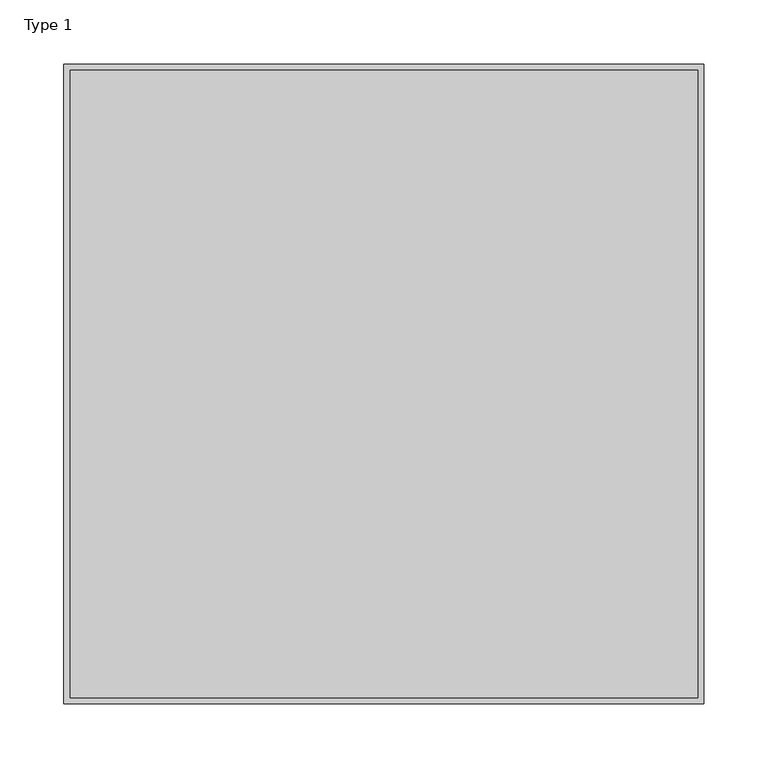
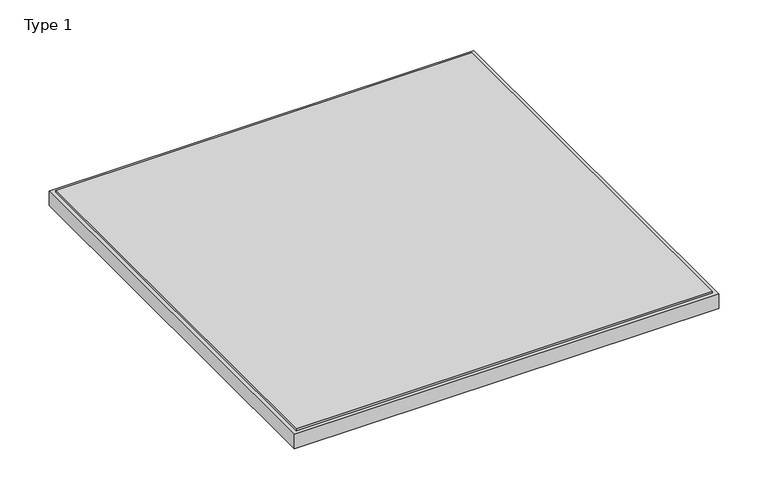
"""IFC4 building model written with IfcOpenShell, lengths in millimetres: plate geometry, 00_CPA_tegel : Type 1."""

from ifc_helpers import new_model, si_unit, origin, origin_with_axes, place, context, project, spatial, polyline, outline, extrude, source, transform, mapped, element, save


def type_1_8eb2385c(model_context):
    return source(origin(), model_context, "Body", "SweptSolid", [
        extrude(outline(polyline([(1000.0, 500.0), (500.0, 500.0), (500.0, 1000.0), (1000.0, 1000.0), (1000.0, 500.0)]), holes=[polyline([(995.0, 995.0), (505.0, 995.0), (505.0, 505.0), (995.0, 505.0), (995.0, 995.0)])]), origin_with_axes(), (0.0, 0.0, 1.0), 18.0),
        extrude(outline(polyline([(505.0, 995.0), (995.0, 995.0), (995.0, 505.0), (505.0, 505.0), (505.0, 995.0)])), origin_with_axes(), (0.0, 0.0, 1.0), 20.0),
    ])


if __name__ == "__main__":
    model = new_model("IFC4")
    model_context = context("Model", 3, world=origin())
    ifc_project = project(units=[si_unit("LENGTHUNIT", "METRE", prefix="MILLI")], contexts=[model_context])
    site = spatial("IfcSite", under=ifc_project)
    building = spatial("IfcBuilding", under=site)
    placement = place(None, origin())
    type_1_shape = type_1_8eb2385c(model_context)
    element("IfcPlate", 1, ObjectType="00_CPA_tegel : Type 1", at=placement, inside=building, context=model_context, shape_type="MappedRepresentation", body=[
        mapped(type_1_shape, transform((0.0, 0.0, 0.0), x_axis=(1.0, 0.0, 0.0), y_axis=(0.0, 1.0, 0.0), z_axis=(0.0, 0.0, 1.0))),
    ])
    save(model, "model.ifc")

# Revit data of these elements
# Type "00_CPA_tegel : Type 1"
#   Voegdikte = 18 mm
#   Tegeldikte = 20 mm
#   HalveVoegbreedte = 5 mm
#   Voeg = 20_voeg
#   MateriaalSteen = 300_hardsteen_zwart
# Element 1 (IfcPlate, "00_CPA_tegel : Type 1")
#   Materials on its faces: "20_voeg", "300_hardsteen_zwart"
# Materials
#   "20_voeg": class "Concrete", colour RGB 86 86 86, transparency 0, Manufacturer = "RevitGG", URL = "www.revitgg.nl", Description = "zandcement, generiek materiaal", Cost = 0
#   "300_hardsteen_zwart": class "Generic", colour RGB 15 15 15, transparency 0, Description = "kalkzandsteen", Cost = 0
